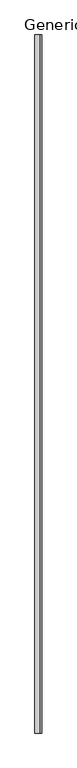
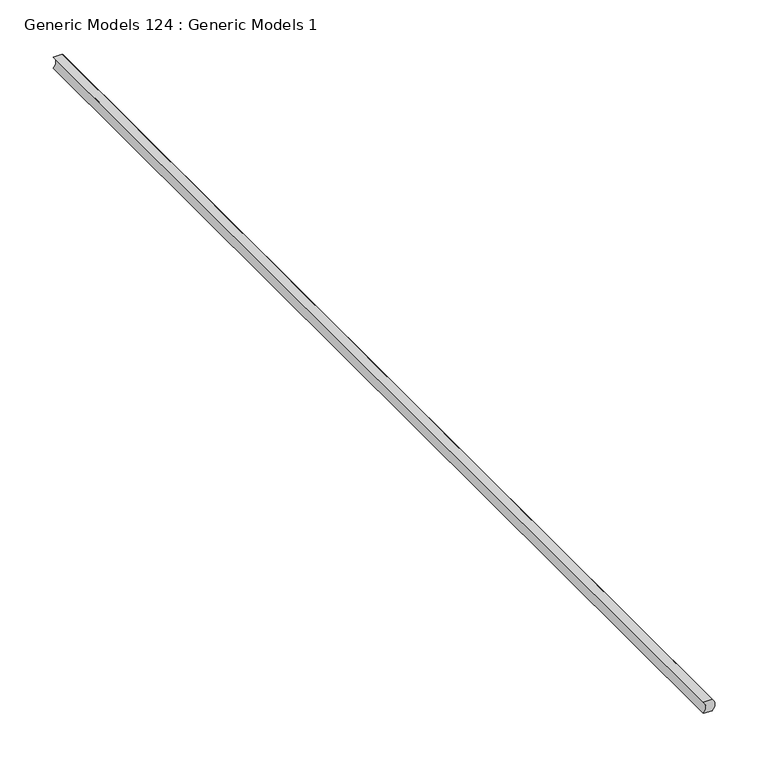
"""IFC4 building model written with IfcOpenShell, lengths in millimetres: proxy geometry, Generic Models 124 : Generic Models 1."""

from ifc_helpers import new_model, si_unit, point, frame, frame_2d, origin, place, context, project, spatial, polyline, circle_curve, trimmed, segment, composite_curve, outline, extrude, source, transform, mapped, element, save


def generic_models_124_generic_models_1_b386a220(model_context):
    return source(origin(), model_context, "Body", "SweptSolid", [
        extrude(outline(composite_curve([segment(polyline([(2218.773933, 49246.8544263), (2218.773933, 49256.3794263)]), True, "CONTINUOUS"), segment(trimmed(circle_curve(frame_2d((2225.123933, 49250.5499453)), 8.620055), [point((2218.773933, 49256.3794263))], [point((2231.473933, 49256.3794263))], False, "CARTESIAN"), True, "CONTINUOUS"), segment(polyline([(2231.473933, 49256.3794263), (2231.473933, 49246.8544263)]), True, "CONTINUOUS"), segment(trimmed(circle_curve(frame_2d((2225.123933, 49241.0249453)), 8.620055), [point((2231.473933, 49246.8544263))], [point((2218.773933, 49246.8544263))], True, "CARTESIAN"), True, "CONTINUOUS")], self_intersect=False)), frame((0.0, 0.0, 0.0), z_axis=(0.0, 1.0, 0.0), x_axis=(0.0, 0.0, 1.0)), (0.0, 0.0, 1.0), 1219.2),
    ])


if __name__ == "__main__":
    model = new_model("IFC4")
    model_context = context("Model", 3, world=origin())
    ifc_project = project(units=[si_unit("LENGTHUNIT", "METRE", prefix="MILLI")], contexts=[model_context])
    site = spatial("IfcSite", under=ifc_project)
    building = spatial("IfcBuilding", under=site)
    placement = place(None, origin())
    generic_models_124_generic_models_1_shape = generic_models_124_generic_models_1_b386a220(model_context)
    element("IfcBuildingElementProxy", 1, Name="Generic Models 124 : Generic Models 1", ObjectType="Generic Models 124 : Generic Models 1", at=placement, inside=building, context=model_context, shape_type="MappedRepresentation", body=[
        mapped(generic_models_124_generic_models_1_shape, transform((0.0, 0.0, 0.0), x_axis=(1.0, 0.0, 0.0), y_axis=(0.0, 1.0, 0.0), z_axis=(0.0, 0.0, 1.0))),
    ])
    save(model, "model.ifc")

# Revit data of these elements
# Element 1 (IfcBuildingElementProxy, "Generic Models 124 : Generic Models 1")
#   Materials on its faces: "SEALANT (W/ BACKER ROD IF NECESSARY)"
# Materials
#   "SEALANT (W/ BACKER ROD IF NECESSARY)": class "Unassigned", colour RGB 120 120 120, transparency 0, Cost = 0
